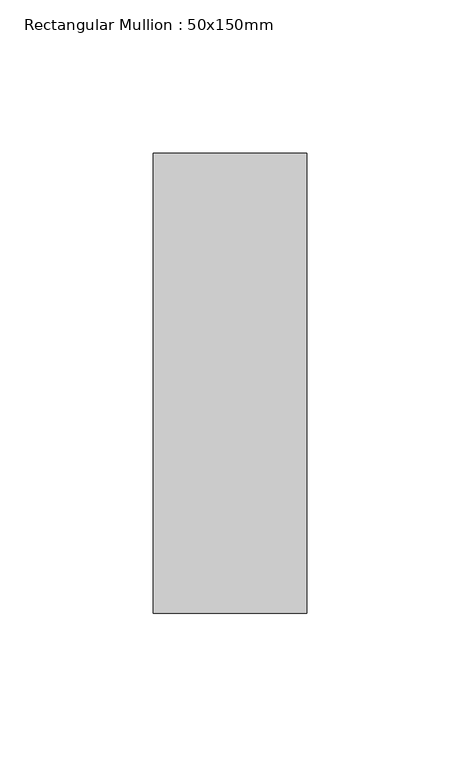
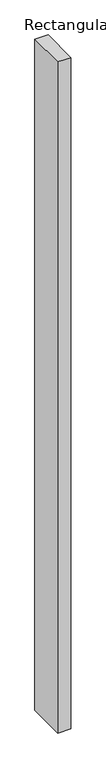
"""IFC4 building model written with IfcOpenShell, lengths in millimetres: member geometry, Rectangular Mullion : 50x150mm."""

from ifc_helpers import new_model, si_unit, frame, origin, place, context, project, spatial, polyline, outline, extrude, source, transform, mapped, element, save


def rectangular_mullion_50x150mm_cf0a7a0a(model_context):
    return source(origin(), model_context, "Body", "SweptSolid", [
        extrude(outline(polyline([(25.0, 75.0), (25.0, -75.0), (-25.0, -75.0), (-25.0, 75.0), (25.0, 75.0)])), frame((0.0, 0.0, -2700.0), z_axis=(0.0, 0.0, 1.0), x_axis=(1.0, 0.0, 0.0)), (0.0, 0.0, 1.0), 2700.0),
    ])


if __name__ == "__main__":
    model = new_model("IFC4")
    model_context = context("Model", 3, world=origin())
    ifc_project = project(units=[si_unit("LENGTHUNIT", "METRE", prefix="MILLI")], contexts=[model_context])
    site = spatial("IfcSite", under=ifc_project)
    building = spatial("IfcBuilding", under=site)
    placement = place(None, origin())
    rectangular_mullion_50x150mm_shape = rectangular_mullion_50x150mm_cf0a7a0a(model_context)
    element("IfcMember", 1, ObjectType="Rectangular Mullion : 50x150mm", at=placement, inside=building, context=model_context, shape_type="MappedRepresentation", body=[
        mapped(rectangular_mullion_50x150mm_shape, transform((0.0, 0.0, 0.0), x_axis=(1.0, 0.0, 0.0), y_axis=(0.0, 1.0, 0.0), z_axis=(0.0, 0.0, 1.0))),
    ])
    save(model, "model.ifc")

# Revit data of these elements
# Type "Rectangular Mullion : 50x150mm"
#   Keynote = "H11"
#   built-in parameter 1007304 = 0.492126 (stored number, unit not read)
#   built-in parameter 1007301 = 0.082021 (stored number, unit not read)
#   built-in parameter 1007300 = 0.082021 (stored number, unit not read)
# Element 1 (IfcMember, "Rectangular Mullion : 50x150mm")
#   Materials on its faces: "Aluminium"
# Materials
#   "Aluminium": class "Metal", colour RGB 247 247 247, transparency 0, Description = "Aluminium 6061", Cost = 0
